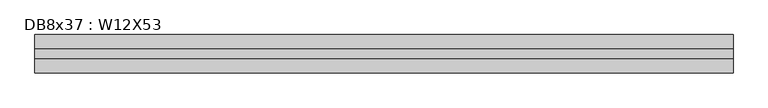
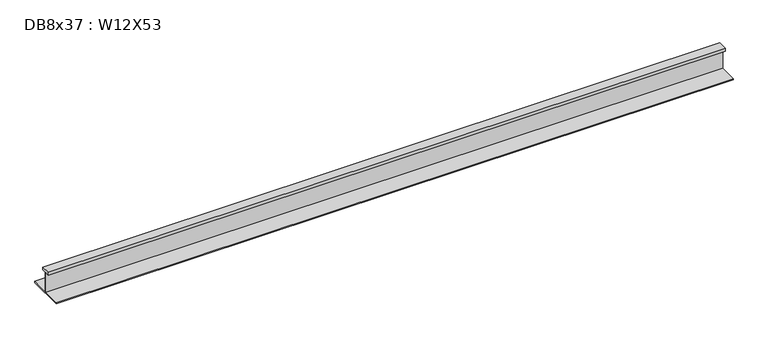
"""IFC4 building model written with IfcOpenShell, lengths in millimetres: beam geometry, DB8x37 : W12X53."""

from ifc_helpers import new_model, si_unit, frame, origin, place, context, project, spatial, polyline, outline, extrude, source, transform, mapped, element, save


def db8x37_w12x53_d3b1ed56(model_context):
    return source(origin(), model_context, "Body", "SweptSolid", [
        extrude(outline(polyline([(38.1, 145.415), (38.1, 120.015), (2.921, 120.015), (2.921, -48.4505), (152.4, -48.4505), (152.4, -58.1025), (-152.4, -58.1025), (-152.4, -48.4505), (-2.921, -48.4505), (-2.921, 120.015), (-38.1, 120.015), (-38.1, 145.415), (38.1, 145.415)])), frame((-2708.529, 0.0, 0.0), z_axis=(1.0, 0.0, 0.0), x_axis=(0.0, 1.0, 0.0)), (0.0, 0.0, 1.0), 5540.6289994),
    ])


if __name__ == "__main__":
    model = new_model("IFC4")
    model_context = context("Model", 3, world=origin())
    ifc_project = project(units=[si_unit("LENGTHUNIT", "METRE", prefix="MILLI")], contexts=[model_context])
    site = spatial("IfcSite", under=ifc_project)
    building = spatial("IfcBuilding", under=site)
    placement = place(None, origin())
    db8x37_w12x53_shape = db8x37_w12x53_d3b1ed56(model_context)
    element("IfcBeam", 1, ObjectType="DB8x37 : W12X53", at=placement, inside=building, context=model_context, shape_type="MappedRepresentation", body=[
        mapped(db8x37_w12x53_shape, transform((0.0, 0.0, 0.0), x_axis=(1.0, 0.0, 0.0), y_axis=(0.0, 1.0, 0.0), z_axis=(0.0, 0.0, 1.0))),
    ])
    save(model, "model.ifc")

# Revit data of these elements
# Type "DB8x37 : W12X53"
#   Assembly Code = "B10"
#   W = 53
#   Length [instance default] = 5' - 0"
#   bf = 0' - 10"
#   d = 1' - 0.1"
#   k = 0' - 1 3/8"
#   k2 = 0' - 0.8"
#   tf = 0' - 0.575"
#   tw = 0' - 0.345"
#   A = 0.108333 SF
#   Structural Material [instance default] = Steel ASTM A992
# Element 1 (IfcBeam, "DB8x37 : W12X53")
#   Materials on its faces: "Steel ASTM A992"
# Materials
#   "Steel ASTM A992": class "Metal", colour RGB 199 199 199, transparency 0, Description = "Structural steel 50ksi", Cost = 0
